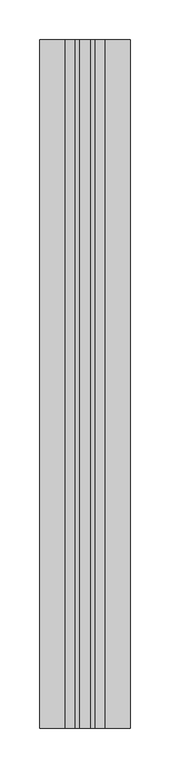
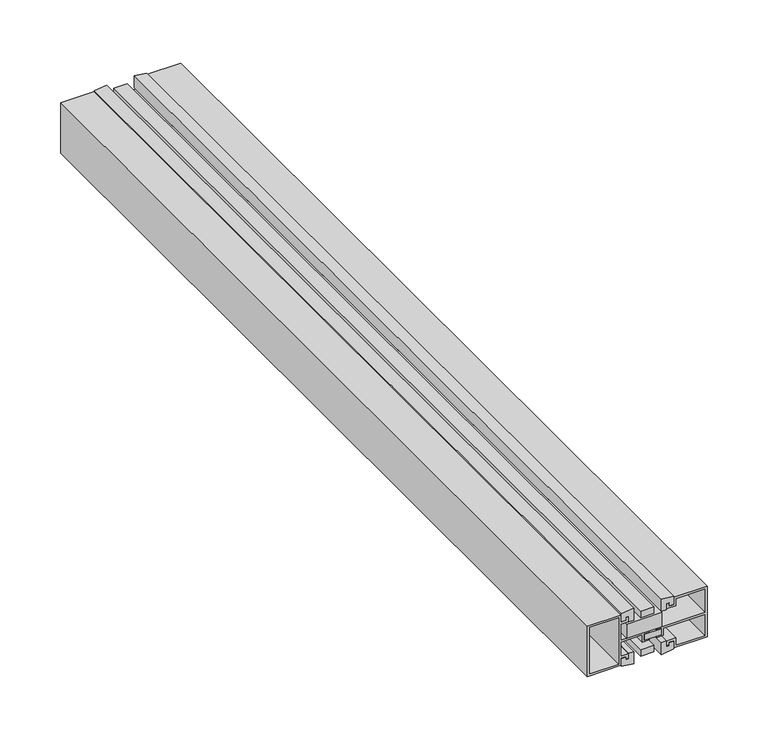
"""IFC4 building model written with IfcOpenShell, lengths in millimetres: proxy geometry, Generic Models 3:Generic Models 1:3:Generic Models 1:3 : Generic Models 3:Generic Models 1:300625:336034:Generic Models 1:3:Generic Models 1:3 : Generic Models 3:Generic Models 1:300625:336034 : Generic Models 3:Generic Models 1:3:Generic Models 1:3 : Generic Models 3:Generic Models 1:300625:336034:2 : Generic Models 3:Generic Models 1:3:Generic Models 1:3 : Generic Models 3:Generic Models 1:300625:336034:Generic Models 1:3:Generic Models 1:3 : Generic Models 3:Generic Models 1:300625:336034 : Generic Models 3:Generic Models 1:3:Generic Models 1:3 : Generic Models 3:Generic Models 1:300625:336034:301191."""

import ifcopenshell
import ifcopenshell.guid

model = None  # the IFC model being written
_history = None  # IfcOwnerHistory: only IFC2X3 demands one
_inside = {}  # id of a spatial element -> (the spatial element, [elements in it])
_under = {}  # id of a project, library or spatial element -> (it, [spatial elements below it])
_declared = {}  # id of a project -> (the project, [libraries it declares])
_typed = {}  # id of a type object -> (the type object, [elements of that type])
_made_of = {}  # id of a material, layer set ... -> (it, [elements and type objects made of it])


def new_model(schema):
    """Start an empty IFC model of exactly this schema.

    Asked for "IFC4X3", IfcOpenShell would pick the latest addendum, in which some entities
    have other attributes; the version numbers below select the first issue.
    IFC2X3 requires an IfcOwnerHistory on every rooted entity: one is made here for all.
    """
    global model, _history
    if schema == "IFC4X3":
        model = ifcopenshell.file(schema_version=(4, 3, 0, 0))
    else:
        model = ifcopenshell.file(schema=schema)
    _inside.clear()
    _under.clear()
    _declared.clear()
    _typed.clear()
    _made_of.clear()
    _history = None
    if model.schema == "IFC2X3":
        org = make("IfcOrganization", Name="unknown")
        user = make(
            "IfcPersonAndOrganization",
            ThePerson=make("IfcPerson", FamilyName="unknown"),
            TheOrganization=org,
        )
        app = make(
            "IfcApplication",
            ApplicationDeveloper=org,
            Version="unknown",
            ApplicationFullName="unknown",
            ApplicationIdentifier="unknown",
        )
        _history = make(
            "IfcOwnerHistory",
            OwningUser=user,
            OwningApplication=app,
            ChangeAction="ADDED",
            CreationDate=0,
        )
    return model


def make(cls, **values):
    """One entity of the class cls with the attributes given. An attribute that is None is left unset."""
    return model.create_entity(
        cls, **{name: value for name, value in values.items() if value is not None}
    )


def rooted(cls, **values):
    """An entity with a GlobalId (a new one), such as an element, a storey or a relation."""
    return make(cls, GlobalId=ifcopenshell.guid.new(), OwnerHistory=_history, **values)


def si_unit(unit_type, name, prefix=None):
    """IfcSIUnit, for example si_unit("LENGTHUNIT", "METRE", prefix="MILLI")."""
    return make("IfcSIUnit", UnitType=unit_type, Prefix=prefix, Name=name)


def assignment(units):
    """IfcUnitAssignment: the units of a project."""
    return None if units is None else make("IfcUnitAssignment", Units=units)


def point(xyz):
    """IfcCartesianPoint."""
    return None if xyz is None else make("IfcCartesianPoint", Coordinates=xyz)


def direction(xyz):
    """IfcDirection."""
    return None if xyz is None else make("IfcDirection", DirectionRatios=xyz)


def frame(location, z_axis=None, x_axis=None):
    """IfcAxis2Placement3D, a coordinate frame: its origin and axes. An axis left out is left unset."""
    return make(
        "IfcAxis2Placement3D",
        Location=point(location),
        Axis=direction(z_axis),
        RefDirection=direction(x_axis),
    )


def origin():
    """The frame at (0, 0, 0) with its axes left unset."""
    return frame((0.0, 0.0, 0.0))


def place(relative_to, where):
    """IfcLocalPlacement: puts the frame where relative to a parent placement (None: the world)."""
    return make(
        "IfcLocalPlacement", PlacementRelTo=relative_to, RelativePlacement=where
    )


def context(
    kind, dimensions, precision=None, world=None, true_north=None, identifier=None
):
    """IfcGeometricRepresentationContext, for example the 3D "Model" context."""
    return make(
        "IfcGeometricRepresentationContext",
        ContextIdentifier=identifier,
        ContextType=kind,
        CoordinateSpaceDimension=dimensions,
        Precision=precision,
        WorldCoordinateSystem=world,
        TrueNorth=true_north,
    )


def project(units=None, contexts=None):
    """IfcProject with its units and contexts."""
    return rooted(
        "IfcProject",
        Name="project",
        RepresentationContexts=contexts,
        UnitsInContext=assignment(units),
    )


def spatial(cls, under=None, at=None, **own):
    """A site, building, storey or space (cls), placed at a placement, below another one or the project."""
    s = rooted(cls, ObjectPlacement=at, **own)
    if under is not None:
        _under.setdefault(under.id(), (under, []))[1].append(s)
    return s


def polyline(points):
    """IfcPolyline through the points."""
    return make("IfcPolyline", Points=[point(p) for p in points])


def outline(outer, holes=None, kind="AREA"):
    """IfcArbitraryClosedProfileDef: a profile drawn as a closed curve; with holes, ...WithVoids."""
    if holes is None:
        return make("IfcArbitraryClosedProfileDef", ProfileType=kind, OuterCurve=outer)
    return make(
        "IfcArbitraryProfileDefWithVoids",
        ProfileType=kind,
        OuterCurve=outer,
        InnerCurves=holes,
    )


def extrude(swept, where, along, depth):
    """IfcExtrudedAreaSolid: the profile swept, set in the frame where, extruded along a direction by depth."""
    return make(
        "IfcExtrudedAreaSolid",
        SweptArea=swept,
        Position=where,
        ExtrudedDirection=direction(along),
        Depth=depth,
    )


def shape(context_of_items, identifier, shape_type, items):
    """IfcShapeRepresentation: the items that make up one representation, for example the "Body"."""
    return make(
        "IfcShapeRepresentation",
        ContextOfItems=context_of_items,
        RepresentationIdentifier=identifier,
        RepresentationType=shape_type,
        Items=items,
    )


def source(mapping_origin, context_of_items, identifier, shape_type, items):
    """IfcRepresentationMap: a shape defined once, which mapped items show again and again."""
    return make(
        "IfcRepresentationMap",
        MappingOrigin=mapping_origin,
        MappedRepresentation=shape(context_of_items, identifier, shape_type, items),
    )


def transform(
    local_origin,
    x_axis=None,
    y_axis=None,
    z_axis=None,
    scale=None,
    scale2=None,
    scale3=None,
    uniform=True,
):
    """IfcCartesianTransformationOperator3D, or its non-uniform kind. x_axis, y_axis, z_axis: its Axis1, 2, 3."""
    if uniform:
        return make(
            "IfcCartesianTransformationOperator3D",
            Axis1=direction(x_axis),
            Axis2=direction(y_axis),
            LocalOrigin=point(local_origin),
            Scale=scale,
            Axis3=direction(z_axis),
        )
    return make(
        "IfcCartesianTransformationOperator3DnonUniform",
        Axis1=direction(x_axis),
        Axis2=direction(y_axis),
        LocalOrigin=point(local_origin),
        Scale=scale,
        Axis3=direction(z_axis),
        Scale2=scale2,
        Scale3=scale3,
    )


def mapped(mapping_source, mapping_target):
    """IfcMappedItem: shows the shape of a source again, moved by a transform."""
    return make(
        "IfcMappedItem", MappingSource=mapping_source, MappingTarget=mapping_target
    )


def made_of(thing, what):
    """Note that an element or type object is made of a material, layer set ...; save() writes the relation."""
    if what is not None:
        _made_of.setdefault(what.id(), (what, []))[1].append(thing)
    return thing


def element(
    cls,
    number,
    at=None,
    inside=None,
    cuts=None,
    type_object=None,
    material=None,
    context=None,
    identifier="Body",
    shape_type=None,
    held_by="IfcProductDefinitionShape",
    body=None,
    shapes=None,
    **own,
):
    """One element of the class cls, such as IfcWall. Its Tag is "e" and its number.

    at: its placement. inside: the storey or other place that contains it. cuts: it is an
    opening in that element (IfcRelVoidsElement). A single representation is given by context,
    identifier, shape_type and body (its items); several are given by shapes. held_by: the class
    of the entity that holds the representations. save() writes the other relations.
    """
    e = rooted(cls, Tag="e%d" % number, ObjectPlacement=at, **own)
    if body is not None:
        shapes = [shape(context, identifier, shape_type, body)]
    if shapes is not None:
        e.Representation = make(held_by, Representations=shapes)
    if inside is not None:
        _inside.setdefault(inside.id(), (inside, []))[1].append(e)
    if cuts is not None:
        rooted(
            "IfcRelVoidsElement", RelatingBuildingElement=cuts, RelatedOpeningElement=e
        )
    if type_object is not None:
        _typed.setdefault(type_object.id(), (type_object, []))[1].append(e)
    return made_of(e, material)


def aggregate(whole, parts):
    """IfcRelAggregates: a whole, such as a stair, and the parts it consists of."""
    return rooted("IfcRelAggregates", RelatingObject=whole, RelatedObjects=parts)


def save(model, path):
    """Write the relations noted so far, then the file.

    IfcRelAggregates (storeys below a building ...), IfcRelContainedInSpatialStructure (elements
    in a storey), IfcRelDefinesByType, IfcRelAssociatesMaterial and IfcRelDeclares: one each for
    every whole, place, type object, material and project.
    """
    for whole, parts in _under.values():
        aggregate(whole, parts)
    for where, things in _inside.values():
        rooted(
            "IfcRelContainedInSpatialStructure",
            RelatedElements=things,
            RelatingStructure=where,
        )
    for kind, things in _typed.values():
        rooted("IfcRelDefinesByType", RelatedObjects=things, RelatingType=kind)
    for what, things in _made_of.values():
        rooted("IfcRelAssociatesMaterial", RelatedObjects=things, RelatingMaterial=what)
    for by, libraries in _declared.values():
        rooted("IfcRelDeclares", RelatingContext=by, RelatedDefinitions=libraries)
    model.write(path)


def generic_models_aaff98bf(model_context):
    return source(origin(), model_context, "Body", "SweptSolid", [
        extrude(outline(polyline([(560311.6698356, -573515.9126607), (560298.9698356, -573515.9126607), (560298.9698356, -572647.5501607), (560311.6698356, -572647.5501607), (560311.6698356, -573515.9126607)])), frame((0.0, 0.0, 2441.2521298), z_axis=(0.0, 0.0, 1.0), x_axis=(1.0, 0.0, 0.0)), (0.0, 0.0, 1.0), 6.3435484),
        extrude(outline(polyline([(2437.3831629, 560280.3335989), (2435.9222961, 560292.2314048), (2447.9925532, 560292.2314048), (2447.9925532, 560287.4773489), (2442.2790126, 560287.4773489), (2442.2790126, 560284.6316707), (2445.2228723, 560284.6316707), (2445.2228723, 560280.3335989), (2437.3831629, 560280.3335989)])), frame((0.0, -573515.9126607, 0.0), z_axis=(0.0, 1.0, 0.0), x_axis=(0.0, 0.0, 1.0)), (0.0, 0.0, 1.0), 868.3625),
        extrude(outline(polyline([(2442.2790126, 560323.1623223), (2447.9925532, 560323.1623223), (2447.9925532, 560318.4082665), (2435.9222961, 560318.4082665), (2437.3831629, 560330.3060723), (2445.2228723, 560330.3060723), (2445.2228723, 560326.0080005), (2442.2790126, 560326.0080005), (2442.2790126, 560323.1623223)])), frame((0.0, -573515.9126607, 0.0), z_axis=(0.0, 1.0, 0.0), x_axis=(0.0, 0.0, 1.0)), (0.0, 0.0, 1.0), 868.3625),
        extrude(outline(polyline([(560319.1513516, -573515.9126607), (560285.8645165, -573515.9126607), (560285.8645165, -572647.5501607), (560319.1513516, -572647.5501607), (560319.1513516, -573515.9126607)])), frame((0.0, 0.0, 2463.7831117), z_axis=(0.0, 0.0, 1.0), x_axis=(1.0, 0.0, 0.0)), (0.0, 0.0, 1.0), 14.2115027),
        extrude(outline(polyline([(560318.4673755, -573515.9126607), (560302.3559394, -573515.9126607), (560302.3559394, -572647.5501607), (560318.4673755, -572647.5501607), (560318.4673755, -573515.9126607)])), frame((0.0, 0.0, 2455.803391), z_axis=(0.0, 0.0, 1.0), x_axis=(1.0, 0.0, 0.0)), (0.0, 0.0, 1.0), 6.0797872),
        extrude(outline(polyline([(560311.6698356, -573515.9126607), (560298.9698356, -573515.9126607), (560298.9698356, -572647.5501607), (560311.6698356, -572647.5501607), (560311.6698356, -573515.9126607)])), frame((0.0, 0.0, 2479.9705452), z_axis=(0.0, 0.0, 1.0), x_axis=(1.0, 0.0, 0.0)), (0.0, 0.0, 1.0), 6.3435484),
        extrude(outline(polyline([(2485.2872108, 560287.4773489), (2479.5736702, 560287.4773489), (2479.5736702, 560292.2314048), (2491.6439273, 560292.2314048), (2490.1830605, 560280.3335989), (2482.3433511, 560280.3335989), (2482.3433511, 560284.6316707), (2485.2872108, 560284.6316707), (2485.2872108, 560287.4773489)])), frame((0.0, -573515.9126607, 0.0), z_axis=(0.0, 1.0, 0.0), x_axis=(0.0, 0.0, 1.0)), (0.0, 0.0, 1.0), 868.3625),
        extrude(outline(polyline([(2490.1830605, 560330.3060723), (2491.6439273, 560318.4082665), (2479.5736702, 560318.4082665), (2479.5736702, 560323.1623223), (2485.2872108, 560323.1623223), (2485.2872108, 560326.0080005), (2482.3433511, 560326.0080005), (2482.3433511, 560330.3060723), (2490.1830605, 560330.3060723)])), frame((0.0, -573515.9126607, 0.0), z_axis=(0.0, 1.0, 0.0), x_axis=(0.0, 0.0, 1.0)), (0.0, 0.0, 1.0), 868.3625),
        extrude(outline(polyline([(2438.4, 560248.1867239), (2438.4, 560279.9367239), (2445.6197473, 560279.9367239), (2445.6197473, 560285.0285457), (2443.1005159, 560285.0285457), (2443.1005159, 560287.0804739), (2447.6716755, 560287.0804739), (2447.6716755, 560279.9367239), (2461.8831782, 560279.9367239), (2461.8831782, 560300.4560059), (2454.5114362, 560300.4560059), (2454.5114362, 560307.2197691), (2455.803391, 560307.2197691), (2455.803391, 560302.3559394), (2461.8831782, 560302.3559394), (2461.8831782, 560307.2197691), (2463.7831117, 560307.2197691), (2463.7831117, 560279.9367239), (2479.9705452, 560279.9367239), (2479.9705452, 560287.0804739), (2484.8903358, 560287.0804739), (2484.8903358, 560285.0285457), (2481.9464761, 560285.0285457), (2481.9464761, 560279.9367239), (2489.1662234, 560279.9367239), (2489.1662234, 560248.1867239), (2438.4, 560248.1867239)]), holes=[polyline([(2487.2662899, 560278.0367904), (2440.2999335, 560278.0367904), (2440.2999335, 560250.6946362), (2487.2662899, 560250.6946362), (2487.2662899, 560278.0367904)])]), frame((0.0, -573515.9126607, 0.0), z_axis=(0.0, 1.0, 0.0), x_axis=(0.0, 0.0, 1.0)), (0.0, 0.0, 1.0), 868.3625),
        extrude(outline(polyline([(2484.8903358, 560325.6111255), (2484.8903358, 560323.5591973), (2479.9705452, 560323.5591973), (2479.9705452, 560332.6028808), (2487.2564243, 560332.6028808), (2487.2564243, 560360.5107931), (2463.7831117, 560360.5107931), (2463.7831117, 560313.6035457), (2461.8831782, 560313.6035457), (2461.8831782, 560318.4673755), (2455.803391, 560318.4673755), (2455.803391, 560313.6035457), (2454.5114362, 560313.6035457), (2454.5114362, 560320.367309), (2461.8831782, 560320.367309), (2461.8831782, 560360.5107931), (2440.3222126, 560360.5107931), (2440.3222126, 560332.6028808), (2447.6716755, 560332.6028808), (2447.6716755, 560323.5591973), (2443.1005159, 560323.5591973), (2443.1005159, 560325.6111255), (2445.6197473, 560325.6111255), (2445.6197473, 560330.7029473), (2438.4, 560330.7029473), (2438.4, 560362.4867239), (2489.1662234, 560362.4867239), (2489.1662234, 560330.7029473), (2481.9464761, 560330.7029473), (2481.9464761, 560325.6111255), (2484.8903358, 560325.6111255)])), frame((0.0, -573515.9126607, 0.0), z_axis=(0.0, 1.0, 0.0), x_axis=(0.0, 0.0, 1.0)), (0.0, 0.0, 1.0), 868.3625),
    ])


if __name__ == "__main__":
    model = new_model("IFC4")
    model_context = context("Model", 3, world=origin())
    ifc_project = project(units=[si_unit("LENGTHUNIT", "METRE", prefix="MILLI")], contexts=[model_context])
    site = spatial("IfcSite", under=ifc_project)
    building = spatial("IfcBuilding", under=site)
    placement = place(None, origin())
    generic_models_shape = generic_models_aaff98bf(model_context)
    element("IfcBuildingElementProxy", 1, Name="Generic Models 3:Generic Models 1:3:Generic Models 1:3 : Generic Models 3:Generic Models 1:300625:336034:Generic Models 1:3:Generic Models 1:3 : Generic Models 3:Generic Models 1:300625:336034 : Generic Models 3:Generic Models 1:3:Generic Models 1:3 : Generic Models 3:Generic Models 1:300625:336034:2 : Generic Models 3:Generic Models 1:3:Generic Models 1:3 : Generic Models 3:Generic Models 1:300625:336034:Generic Models 1:3:Generic Models 1:3 : Generic Models 3:Generic Models 1:300625:336034 : Generic Models 3:Generic Models 1:3:Generic Models 1:3 : Generic Models 3:Generic Models 1:300625:336034:301191", ObjectType="Generic Models 3:Generic Models 1:3:Generic Models 1:3 : Generic Models 3:Generic Models 1:300625:336034:Generic Models 1:3:Generic Models 1:3 : Generic Models 3:Generic Models 1:300625:336034 : Generic Models 3:Generic Models 1:3:Generic Models 1:3 : Generic Models 3:Generic Models 1:300625:336034:2 : Generic Models 3:Generic Models 1:3:Generic Models 1:3 : Generic Models 3:Generic Models 1:300625:336034:Generic Models 1:3:Generic Models 1:3 : Generic Models 3:Generic Models 1:300625:336034 : Generic Models 3:Generic Models 1:3:Generic Models 1:3 : Generic Models 3:Generic Models 1:300625:336034:301191", at=placement, inside=building, context=model_context, shape_type="MappedRepresentation", body=[
        mapped(generic_models_shape, transform((0.0, 0.0, 0.0), x_axis=(1.0, 0.0, 0.0), y_axis=(0.0, 1.0, 0.0), z_axis=(0.0, 0.0, 1.0))),
    ])
    save(model, "model.ifc")

# Revit data of these elements
# Type "Generic Models 3:Generic Models 1:3:Generic Models 1:3 : Generic Models 3:Generic Models 1:300625:336034:Generic Models 1:3:Generic Models 1:3 : Generic Models 3:Generic Models 1:300625:336034 : Generic Models 3:Generic Models 1:3:Generic Models 1:3 : Generic Models 3:Generic Models 1:300625:336034:2 : Generic Models 3:Generic Models 1:3:Generic Models 1:3 : Generic Models 3:Generic Models 1:300625:336034:Generic Models 1:3:Generic Models 1:3 : Generic Models 3:Generic Models 1:300625:336034 : Generic Models 3:Generic Models 1:3:Generic Models 1:3 : Generic Models 3:Generic Models 1:300625:336034:301191"
#   NameOverride = "Generic Models 3:Generic Models 1:3:Generic Models 1:3 : Generic Models 3:Generic Models 1:300625:336034:Generic Models 1:3:Generic Models 1:3 : Generic Models 3:Generic Models 1:300625:336034 : Generic Models 3:Generic Models 1:3:Generic Models 1:3 : Generic Models 3:Generic Models 1:300625:336034:301191"
#   ObjectTypeOverride = "Generic Models 1:3:Generic Models 1:3 : Generic Models 3:Generic Models 1:300625:336034 : Generic Models 3:Generic Models 1:3:Generic Models 1:3 : Generic Models 3:Generic Models 1:300625:336034"
#   Reference = "Generic Models 1"
#   Tag = "301191"
# Element 1 (IfcBuildingElementProxy, "Generic Models 3:Generic Models 1:3:Generic Models 1:3 : Generic Models 3:Generic Models 1:300625:336034:Generic Models 1:3:Generic Models 1:3 : Generic Models 3:Generic Models 1:300625:336034 : Generic Models 3:Generic Models 1:3:Generic Models 1:3 : Generic Models 3:Generic Models 1:300625:336034:2 : Generic Models 3:Generic Models 1:3:Generic Models 1:3 : Generic Models 3:Generic Models 1:300625:336034:Generic Models 1:3:Generic Models 1:3 : Generic Models 3:Generic Models 1:300625:336034 : Generic Models 3:Generic Models 1:3:Generic Models 1:3 : Generic Models 3:Generic Models 1:300625:336034:301191")
#   Materials on its faces: "THERMAL BROKEN ALUMINUM STOREFRONT", "Compression Gasket_1", "Desiccant Sealant_1"
# Materials
#   "THERMAL BROKEN ALUMINUM STOREFRONT": class "Unassigned", colour RGB 244 244 244, transparency 0, Cost = 0
#   "Compression Gasket_1": class "Unassigned", colour RGB 178 178 178, transparency 0
#   "Desiccant Sealant_1": class "Unassigned", colour RGB 120 120 120, transparency 0
